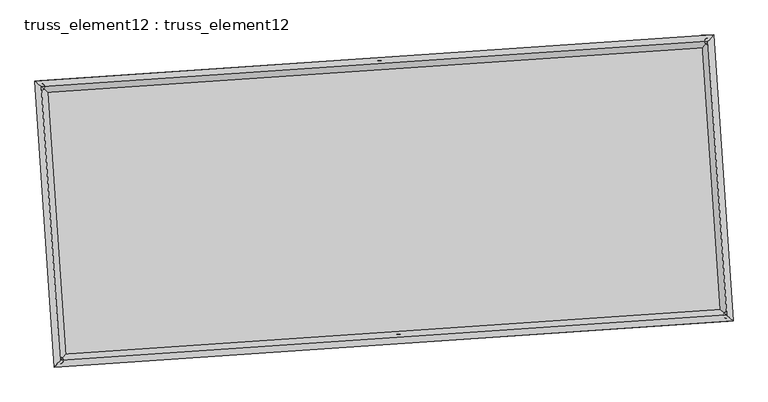
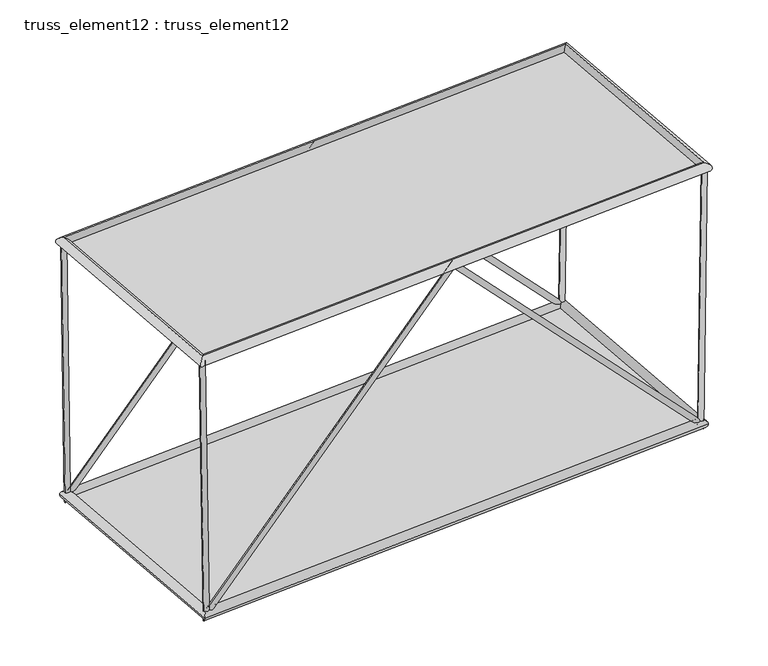
"""IFC4 building model written with IfcOpenShell, lengths in millimetres: plate geometry, truss_element12 : truss_element12."""

from ifc_helpers import new_model, si_unit, frame, origin, origin_with_axes, place, context, project, spatial, polyline, circle_curve, ellipse_curve, outline, extrude, source, transform, mapped, element, save
from ifc_brep_helpers import plane_surface, cylinder_surface, advanced_brep


def truss_element12_truss_element12_84eb71f0(model_context):
    return source(origin(), model_context, "Body", "SolidModel", [
        advanced_brep(
        [(-3738.1719305, 2271.2306691, 5000.1936445), (-3837.2645722, 2257.8701682, 4998.7289371), (-3666.7279155, 2276.1021649, 122.3170416), (-3762.2589673, 2262.9845152, -122.3170416), (1064.3804655, 2598.6984607, 5071.5713816), (1064.8187958, 2592.1245985, 4927.3317181), (5794.1985434, 2921.2067757, 122.3079006), (5890.5624336, 2921.1737128, -122.3079006), (5866.9231849, 2926.1655926, 5000.1872867), (5966.9118404, 2926.3796886, 4998.6963313)],
        [
            (0, 1, circle_curve(frame((-3787.7182514, 2264.5504186, 4999.4612908), z_axis=(-0.014644961991441706, -0.0009985842874851005, 0.9998922581546924), x_axis=(-0.13360524041134672, 0.9910341590580329, -0.0009671167270260404)), 50.0)),
            (1, 0, circle_curve(frame((-3787.7182514, 2264.5504186, 4999.4612908), z_axis=(-0.014644961991441706, -0.0009985842874851005, 0.9998922581546924), x_axis=(-0.13360524041134672, 0.9910341590580329, -0.0009671167270260404)), 50.0)),
            (0, 2),
            (2, 3, ellipse_curve(frame((-3714.4934414, 2269.54334, 0.0), z_axis=(-0.9284714273096889, -0.0633089371779296, 0.36596828707267776), x_axis=(0.3651204835023745, 0.02489617781712952, 0.9306273222171646)), 131.7212392, 50.0)),
            (3, 1),
            (3, 2, ellipse_curve(frame((-3714.4934414, 2269.54334, 0.0), z_axis=(-0.9284714273096889, -0.0633089371779296, 0.36596828707267776), x_axis=(0.3651204835023745, 0.02489617781712952, 0.9306273222171646)), 131.7212392, 50.0)),
            (2, 4),
            (4, 5, ellipse_curve(frame((1064.5996306, 2595.4115296, 4999.4515499), z_axis=(-0.9976833937280466, -0.06802823806868141, 6.85897849258551e-05), x_axis=(-6.843088956082228e-05, -4.66604222811254e-06, -0.9999999976477207)), 72.2768712, 50.0)),
            (5, 3),
            (5, 4, ellipse_curve(frame((1064.5996306, 2595.4115296, 4999.4515499), z_axis=(-0.9976833937280466, -0.06802823806868141, 6.85897849258551e-05), x_axis=(-6.843088956082228e-05, -4.66604222811254e-06, -0.9999999976477207)), 72.2768712, 50.0)),
            (4, 6),
            (6, 7, ellipse_curve(frame((5842.3804885, 2921.1902443, 0.0), z_axis=(-0.9285444803963764, -0.06331391839020893, -0.3657820329971133), x_axis=(-0.3649346609037325, -0.024883507280507755, 0.9307005449318803)), 131.701033, 50.0)),
            (7, 5),
            (7, 6, ellipse_curve(frame((5842.3804885, 2921.1902443, 0.0), z_axis=(-0.9285444803963764, -0.06331391839020893, -0.3657820329971133), x_axis=(-0.3649346609037325, -0.024883507280507755, 0.9307005449318803)), 131.701033, 50.0)),
            (8, 9, circle_curve(frame((5916.9175126, 2926.2726406, 4999.441809), z_axis=(0.014907404826636871, 0.0010164792667763506, 0.999888361794073), x_axis=(-0.002155876072210697, 0.9999971915265048, -0.0009844477966426126)), 50.0)),
            (9, 8, circle_curve(frame((5916.9175126, 2926.2726406, 4999.441809), z_axis=(0.014907404826636871, 0.0010164792667763506, 0.999888361794073), x_axis=(-0.002155876072210697, 0.9999971915265048, -0.0009844477966426126)), 50.0)),
            (6, 8),
            (9, 7),
        ],
        [
            plane_surface(frame((-3787.7182514, 2314.5503937, 4999.5112253), z_axis=(-0.014644961991443045, -0.0009985842874868955, 0.9998922581546923), x_axis=(0.9998927567935819, -1.4625797453149408e-05, 0.014644954688112227))),
            cylinder_surface(frame((-3787.7182514, 2264.5504186, 4999.4612908), z_axis=(-0.014644961991441706, -0.0009985842874851005, 0.9998922581546924), x_axis=(-0.13360524041134672, 0.9910341590580329, -0.0009671167270260404)), 50.0),
            cylinder_surface(frame((-3714.4934414, 2269.54334, 0.0), z_axis=(-0.6902310570943103, -0.04706423196937367, -0.7220568162489739), x_axis=(-0.020418269302223836, 0.998751948354006, -0.04558113576665978)), 50.0),
            cylinder_surface(frame((1064.5996306, 2595.4115296, 4999.4515499), z_axis=(-0.6901322286195789, -0.04705749323136519, 0.7221517149127), x_axis=(-0.11534882893492074, 0.9922789943574934, -0.045574609380925536)), 50.0),
            plane_surface(frame((5916.9175126, 2876.2726664, 4999.4926386), z_axis=(0.014907404826636708, 0.0010164792667773021, 0.999888361794073), x_axis=(0.9998888784666699, -1.5154751947576975e-05, -0.014907397123533164))),
            cylinder_surface(frame((5842.3804885, 2921.1902443, 0.0), z_axis=(-0.014907404826636871, -0.0010164792667763506, -0.999888361794073), x_axis=(-0.002155876072210697, 0.9999971915265048, -0.0009844477966426126)), 50.0),
        ],
        [
            (0, [[1, 2]]),
            (1, [[-1, 3, 4, 5]]),
            (1, [[-2, -5, 6, -3]]),
            (2, [[-4, 7, 8, 9]]),
            (2, [[-6, -9, 10, -7]]),
            (3, [[-8, 11, 12, 13]]),
            (3, [[-10, -13, 14, -11]]),
            (4, [[15, 16]]),
            (5, [[-12, 17, -16, 18]]),
            (5, [[-14, -18, -15, -17]]),
        ],
    ),
        advanced_brep(
        [(-3466.0589776, -1719.5029152, 5000.1936445), (-3565.1516193, -1732.8634161, 4998.7289371), (-3394.6149626, -1714.6314194, 122.3170416), (-3490.1460144, -1727.7490691, -122.3170416), (1336.4934184, -1392.0351236, 5071.5713816), (1336.9317487, -1398.6089858, 4927.3317181), (6066.3114963, -1069.5268086, 122.3079006), (6162.6753866, -1069.5598715, -122.3079006), (6139.0361378, -1064.5679917, 5000.1872867), (6239.0247933, -1064.3538957, 4998.6963313)],
        [
            (0, 1, circle_curve(frame((-3515.6052985, -1726.1831657, 4999.4612908), z_axis=(-0.014644961991442204, -0.0009985842874851928, 0.9998922581546925), x_axis=(-0.13360524041134608, 0.991034159058033, -0.0009671167270260054)), 50.0)),
            (1, 0, circle_curve(frame((-3515.6052985, -1726.1831657, 4999.4612908), z_axis=(-0.014644961991442204, -0.0009985842874851928, 0.9998922581546925), x_axis=(-0.13360524041134608, 0.991034159058033, -0.0009671167270260054)), 50.0)),
            (0, 2),
            (2, 3, ellipse_curve(frame((-3442.3804885, -1721.1902443, 0.0), z_axis=(-0.9284714273096893, -0.06330893717792938, 0.36596828707267676), x_axis=(0.3651204835023735, 0.024896177817129286, 0.9306273222171649)), 131.7212392, 50.0)),
            (3, 1),
            (3, 2, ellipse_curve(frame((-3442.3804885, -1721.1902443, 0.0), z_axis=(-0.9284714273096893, -0.06330893717792938, 0.36596828707267676), x_axis=(0.3651204835023735, 0.024896177817129286, 0.9306273222171649)), 131.7212392, 50.0)),
            (2, 4),
            (4, 5, ellipse_curve(frame((1336.7125835, -1395.3220547, 4999.4515499), z_axis=(-0.9976833937280464, -0.06802823806868134, 6.858978492489223e-05), x_axis=(-6.843088956020724e-05, -4.666042227776212e-06, -0.9999999976477207)), 72.2768712, 50.0)),
            (5, 3),
            (5, 4, ellipse_curve(frame((1336.7125835, -1395.3220547, 4999.4515499), z_axis=(-0.9976833937280464, -0.06802823806868134, 6.858978492489223e-05), x_axis=(-6.843088956020724e-05, -4.666042227776212e-06, -0.9999999976477207)), 72.2768712, 50.0)),
            (4, 6),
            (6, 7, ellipse_curve(frame((6114.4934414, -1069.54334, 0.0), z_axis=(-0.9285444803963764, -0.06331391839020908, -0.36578203299711354), x_axis=(-0.36493466090373267, -0.024883507280507897, 0.9307005449318803)), 131.701033, 50.0)),
            (7, 5),
            (7, 6, ellipse_curve(frame((6114.4934414, -1069.54334, 0.0), z_axis=(-0.9285444803963764, -0.06331391839020908, -0.36578203299711354), x_axis=(-0.36493466090373267, -0.024883507280507897, 0.9307005449318803)), 131.701033, 50.0)),
            (8, 9, circle_curve(frame((6189.0304655, -1064.4609437, 4999.441809), z_axis=(0.01490740482663649, 0.001016479266776253, 0.999888361794073), x_axis=(-0.00215587607221119, 0.9999971915265048, -0.0009844477966425085)), 50.0)),
            (9, 8, circle_curve(frame((6189.0304655, -1064.4609437, 4999.441809), z_axis=(0.01490740482663649, 0.001016479266776253, 0.999888361794073), x_axis=(-0.00215587607221119, 0.9999971915265048, -0.0009844477966425085)), 50.0)),
            (6, 8),
            (9, 7),
        ],
        [
            plane_surface(frame((-3515.6052985, -1676.1831906, 4999.5112253), z_axis=(-0.014644961991443045, -0.0009985842874868955, 0.9998922581546923), x_axis=(0.9998927567935819, -1.4625797453149408e-05, 0.014644954688112227))),
            cylinder_surface(frame((-3515.6052985, -1726.1831657, 4999.4612908), z_axis=(-0.0146449619914422, -0.0009985842874851926, 0.9998922581546923), x_axis=(-0.13360524041134608, 0.991034159058033, -0.0009671167270260054)), 50.0),
            cylinder_surface(frame((-3442.3804885, -1721.1902443, 0.0), z_axis=(-0.6902310570943089, -0.047064231969373316, -0.7220568162489751), x_axis=(-0.020418269302223697, 0.998751948354006, -0.04558113576665939)), 50.0),
            cylinder_surface(frame((1336.7125835, -1395.3220547, 4999.4515499), z_axis=(-0.6901322286195789, -0.04705749323136537, 0.7221517149127), x_axis=(-0.11534882893492066, 0.9922789943574934, -0.04557460938092523)), 50.0),
            plane_surface(frame((6189.0304655, -1114.4609179, 4999.4926386), z_axis=(0.014907404826636708, 0.0010164792667773034, 0.999888361794073), x_axis=(0.9998888784666699, -1.5154751947132886e-05, -0.014907397123533164))),
            cylinder_surface(frame((6114.4934414, -1069.54334, 0.0), z_axis=(-0.01490740482663649, -0.001016479266776253, -0.999888361794073), x_axis=(-0.00215587607221119, 0.9999971915265048, -0.0009844477966425085)), 50.0),
        ],
        [
            (0, [[1, 2]]),
            (1, [[-1, 3, 4, 5]]),
            (1, [[-2, -5, 6, -3]]),
            (2, [[-4, 7, 8, 9]]),
            (2, [[-6, -9, 10, -7]]),
            (3, [[-8, 11, 12, 13]]),
            (3, [[-10, -13, 14, -11]]),
            (4, [[15, 16]]),
            (5, [[-12, 17, -16, 18]]),
            (5, [[-14, -18, -15, -17]]),
        ],
    ),
        advanced_brep(
        [(-3515.6103992, -1726.188819, 4909.4612909), (-3515.6001977, -1726.1775123, 5089.4612906), (-3787.7124305, 2264.54551, 5089.4612906), (-3787.7240723, 2264.5553272, 4909.4612909), (5916.9127716, 2926.2670118, 5089.4418088), (5916.9222537, 2926.2782694, 4909.4418091), (6189.0250043, -1064.4560106, 5089.4418088), (6189.0359268, -1064.4658769, 4909.4418091)],
        [
            (0, 1, ellipse_curve(frame((-3515.6052985, -1726.1831657, 4999.4612908), z_axis=(-0.7535719234040441, 0.6573654662781759, 1.4162100019367173e-06), x_axis=(-0.6573654662766645, -0.7535719234053627, 1.4162099958110949e-06)), 127.2792206, 90.0)),
            (1, 2),
            (2, 3, ellipse_curve(frame((-3787.7182514, 2264.5504186, 4999.4612908), z_axis=(-0.6573654662766646, -0.7535719234053626, 1.4162099970705765e-06), x_axis=(0.7535719234040441, -0.6573654662781759, -1.4162100031961985e-06)), 127.2792206, 90.0)),
            (3, 0),
            (1, 0, ellipse_curve(frame((-3515.6052985, -1726.1831657, 4999.4612908), z_axis=(-0.7535719234040441, 0.6573654662781759, 1.4162100019367173e-06), x_axis=(-0.6573654662766645, -0.7535719234053627, 1.4162099958110949e-06)), 127.2792206, 90.0)),
            (3, 2, ellipse_curve(frame((-3787.7182514, 2264.5504186, 4999.4612908), z_axis=(-0.6573654662766646, -0.7535719234053626, 1.4162099970705765e-06), x_axis=(0.7535719234040441, -0.6573654662781759, -1.4162100031961985e-06)), 127.2792206, 90.0)),
            (2, 4),
            (4, 5, ellipse_curve(frame((5916.9175126, 2926.2726406, 4999.441809), z_axis=(-0.7535719234040424, 0.6573654662781778, 1.4162100001333888e-06), x_axis=(-0.6573654662766668, -0.7535719234053607, 1.4162100001333862e-06)), 127.2792206, 90.0)),
            (5, 3),
            (5, 4, ellipse_curve(frame((5916.9175126, 2926.2726406, 4999.441809), z_axis=(-0.7535719234040424, 0.6573654662781778, 1.4162100001333888e-06), x_axis=(-0.6573654662766668, -0.7535719234053607, 1.4162100001333862e-06)), 127.2792206, 90.0)),
            (4, 6),
            (6, 7, ellipse_curve(frame((6189.0304655, -1064.4609437, 4999.441809), z_axis=(0.6573654662766664, 0.7535719234053609, -1.4162099988739046e-06), x_axis=(-0.7535719234040424, 0.6573654662781779, 1.416209998873908e-06)), 127.2792206, 90.0)),
            (7, 5),
            (7, 6, ellipse_curve(frame((6189.0304655, -1064.4609437, 4999.441809), z_axis=(0.6573654662766664, 0.7535719234053609, -1.4162099988739046e-06), x_axis=(-0.7535719234040424, 0.6573654662781779, 1.416209998873908e-06)), 127.2792206, 90.0)),
            (6, 1),
            (0, 7),
        ],
        [
            cylinder_surface(frame((-3515.6052985, -1726.1831657, 4999.4612908), z_axis=(0.06802823822870303, -0.9976833960748765, 0.0), x_axis=(-0.9976833942298228, -0.06802823810289584, 6.081673841838858e-05)), 90.0),
            cylinder_surface(frame((-3787.7182514, 2264.5504186, 4999.4612908), z_axis=(-0.9976833960728756, -0.06802823822856638, 2.0028233893570394e-06), x_axis=(-0.06802823799352438, 0.9976833943573582, 5.8813915036826964e-05)), 90.0),
            cylinder_surface(frame((5916.9175126, 2926.2726406, 4999.441809), z_axis=(-0.0680282382286981, 0.997683396074877, 0.0), x_axis=(0.9976833944648652, 0.06802823811891752, 5.681109165093387e-05)), 90.0),
            cylinder_surface(frame((6189.0304655, -1064.4609437, 4999.441809), z_axis=(0.9976833960728756, 0.06802823822856637, -2.002823387575864e-06), x_axis=(0.06802823822856635, -0.9976833943413315, 5.8813915035045755e-05)), 90.0),
        ],
        [
            (0, [[1, 2, 3, 4]]),
            (0, [[5, -4, 6, -2]]),
            (1, [[-3, 7, 8, 9]]),
            (1, [[-6, -9, 10, -7]]),
            (2, [[-8, 11, 12, 13]]),
            (2, [[-10, -13, 14, -11]]),
            (3, [[-12, 15, -1, 16]]),
            (3, [[-14, -16, -5, -15]]),
        ],
    ),
        advanced_brep(
        [(-3358.7115243, -1625.2761972, 0.0), (-3526.0494527, -1817.1042913, 0.0), (-3810.4074885, 2353.2123043, 0.0), (-3618.5793943, 2185.8743758, 0.0), (5926.0494527, 3017.1042913, 0.0), (5758.7115243, 2825.2761972, 0.0), (6210.4074885, -1153.2123043, 0.0), (6018.5793943, -985.8743758, 0.0)],
        [
            (0, 1, ellipse_curve(frame((-3442.3804885, -1721.1902443, 0.0), z_axis=(-0.7535719234054591, 0.6573654662780795, 0.0), x_axis=(-0.6573654662780795, -0.7535719234054591, 0.0)), 127.2792206, 90.0)),
            (1, 2),
            (2, 3, ellipse_curve(frame((-3714.4934414, 2269.54334, 0.0), z_axis=(-0.6573654662780796, -0.7535719234054591, 0.0), x_axis=(0.7535719234054591, -0.6573654662780796, 0.0)), 127.2792206, 90.0)),
            (3, 0),
            (1, 0, ellipse_curve(frame((-3442.3804885, -1721.1902443, 0.0), z_axis=(-0.7535719234054591, 0.6573654662780795, 0.0), x_axis=(-0.6573654662780795, -0.7535719234054591, 0.0)), 127.2792206, 90.0)),
            (3, 2, ellipse_curve(frame((-3714.4934414, 2269.54334, 0.0), z_axis=(-0.6573654662780796, -0.7535719234054591, 0.0), x_axis=(0.7535719234054591, -0.6573654662780796, 0.0)), 127.2792206, 90.0)),
            (2, 4),
            (4, 5, ellipse_curve(frame((5842.3804885, 2921.1902443, 0.0), z_axis=(-0.7535719234054576, 0.657365466278081, 0.0), x_axis=(-0.6573654662780813, -0.7535719234054575, 0.0)), 127.2792206, 90.0)),
            (5, 3),
            (5, 4, ellipse_curve(frame((5842.3804885, 2921.1902443, 0.0), z_axis=(-0.7535719234054576, 0.657365466278081, 0.0), x_axis=(-0.6573654662780813, -0.7535719234054575, 0.0)), 127.2792206, 90.0)),
            (4, 6),
            (6, 7, ellipse_curve(frame((6114.4934414, -1069.54334, 0.0), z_axis=(0.6573654662780811, 0.7535719234054578, 0.0), x_axis=(-0.7535719234054578, 0.6573654662780811, 0.0)), 127.2792206, 90.0)),
            (7, 5),
            (7, 6, ellipse_curve(frame((6114.4934414, -1069.54334, 0.0), z_axis=(0.6573654662780811, 0.7535719234054578, 0.0), x_axis=(-0.7535719234054578, 0.6573654662780811, 0.0)), 127.2792206, 90.0)),
            (6, 1),
            (0, 7),
        ],
        [
            cylinder_surface(frame((-3442.3804885, -1721.1902443, 0.0), z_axis=(0.06802823822870317, -0.9976833960748764, 0.0), x_axis=(-0.9976833960748764, -0.06802823822870317, 0.0)), 90.0),
            cylinder_surface(frame((-3714.4934414, 2269.54334, 0.0), z_axis=(-0.9976833960748767, -0.06802823822870281, 0.0), x_axis=(-0.06802823822870281, 0.9976833960748767, 0.0)), 90.0),
            cylinder_surface(frame((5842.3804885, 2921.1902443, 0.0), z_axis=(-0.06802823822869876, 0.9976833960748768, 0.0), x_axis=(0.9976833960748768, 0.06802823822869876, 0.0)), 90.0),
            cylinder_surface(frame((6114.4934414, -1069.54334, 0.0), z_axis=(0.9976833960748764, 0.06802823822870295, 0.0), x_axis=(0.06802823822870295, -0.9976833960748764, 0.0)), 90.0),
        ],
        [
            (0, [[1, 2, 3, 4]]),
            (0, [[5, -4, 6, -2]]),
            (1, [[-3, 7, 8, 9]]),
            (1, [[-6, -9, 10, -7]]),
            (2, [[-8, 11, 12, 13]]),
            (2, [[-10, -13, 14, -11]]),
            (3, [[-12, 15, -1, 16]]),
            (3, [[-14, -16, -5, -15]]),
        ],
    ),
        extrude(outline(polyline([(-3442.3804885, -1721.1902443), (-3714.4934414, 2269.54334), (5842.3804885, 2921.1902443), (6114.4934414, -1069.54334), (-3442.3804885, -1721.1902443)])), origin_with_axes(), (0.0, 0.0, 1.0), 20.0),
        extrude(outline(polyline([(-2000.0, 4863.5848819), (2000.0, 4863.5848819), (2000.0000001, -4863.5848818), (-1999.9999999, -4863.5848818), (-2000.0, 4863.5848819)])), frame((1200.6561071, 600.0447374, 4999.4515499), z_axis=(1.9981836411265887e-06, 1.3624854233976442e-07, 0.9999999999979944), x_axis=(-0.06802823822870277, 0.9976833960748765, 0.0)), (0.0, 0.0, 1.0), 20.0),
    ])


if __name__ == "__main__":
    model = new_model("IFC4")
    model_context = context("Model", 3, world=origin())
    ifc_project = project(units=[si_unit("LENGTHUNIT", "METRE", prefix="MILLI")], contexts=[model_context])
    site = spatial("IfcSite", under=ifc_project)
    building = spatial("IfcBuilding", under=site)
    placement = place(None, origin())
    truss_element12_truss_element12_shape = truss_element12_truss_element12_84eb71f0(model_context)
    element("IfcPlate", 1, ObjectType="truss_element12 : truss_element12", at=placement, inside=building, context=model_context, shape_type="MappedRepresentation", body=[
        mapped(truss_element12_truss_element12_shape, transform((0.0, 0.0, 0.0), x_axis=(1.0, 0.0, 0.0), y_axis=(0.0, 1.0, 0.0), z_axis=(0.0, 0.0, 1.0))),
    ])
    save(model, "model.ifc")

# Revit data of these elements
# Type "truss_element12 : truss_element12"
#   steellbar1 = 90 mm
#   steelbar2 = 50 mm
#   offset1 = 5000 mm
#   M = Default Roof
# Element 1 (IfcPlate, "truss_element12 : truss_element12")
#   Materials on its faces: "Default Roof"
# Materials
#   "Default Roof": class "Miscellaneous", colour RGB 0 127 0, transparency 0, Comments = "Rendering appearance not upgraded Rendering appearance not upgraded ", Cost = 0
